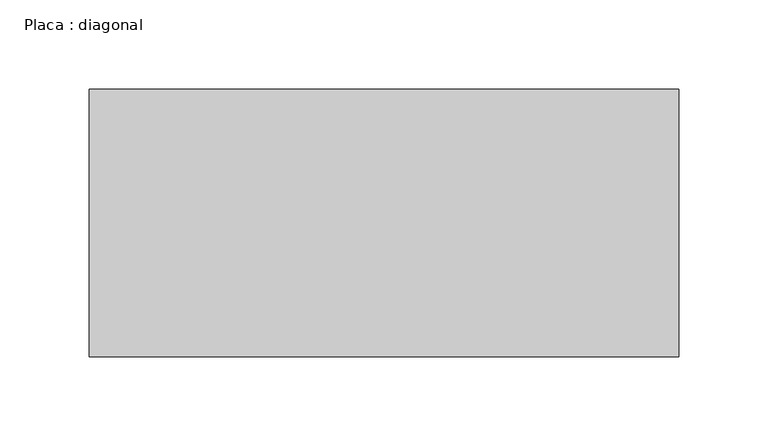
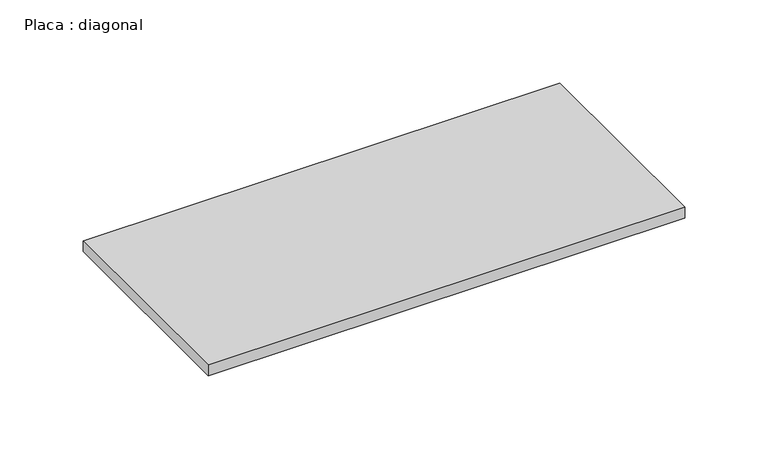
"""IFC4 building model written with IfcOpenShell, lengths in millimetres: beam geometry, Placa : diagonal."""

from ifc_helpers import new_model, si_unit, frame, origin, place, context, project, spatial, polyline, outline, extrude, source, transform, mapped, element, save


def placa_diagonal_d62ed6d6(model_context):
    return source(origin(), model_context, "Body", "SweptSolid", [
        extrude(outline(polyline([(165.4962734, 75.0), (165.4962734, -75.0), (-165.170522, -75.0), (-165.170522, 75.0), (165.4962734, 75.0)])), frame((0.0, 0.0, -4.0), z_axis=(0.0, 0.0, 1.0), x_axis=(1.0, 0.0, 0.0)), (0.0, 0.0, 1.0), 8.0),
    ])


if __name__ == "__main__":
    model = new_model("IFC4")
    model_context = context("Model", 3, world=origin())
    ifc_project = project(units=[si_unit("LENGTHUNIT", "METRE", prefix="MILLI")], contexts=[model_context])
    site = spatial("IfcSite", under=ifc_project)
    building = spatial("IfcBuilding", under=site)
    placement = place(None, origin())
    placa_diagonal_shape = placa_diagonal_d62ed6d6(model_context)
    element("IfcBeam", 1, ObjectType="Placa : diagonal", at=placement, inside=building, context=model_context, shape_type="MappedRepresentation", body=[
        mapped(placa_diagonal_shape, transform((0.0, 0.0, 0.0), x_axis=(1.0, 0.0, 0.0), y_axis=(0.0, 1.0, 0.0), z_axis=(0.0, 0.0, 1.0))),
    ])
    save(model, "model.ifc")

# Revit data of these elements
# Type "Placa : diagonal"
#   W = 0
#   Length [instance default] = 1.50 m
#   b = 0.15 m
#   d = 0.008 m
#   A = 0 m²
#   Structural Material [instance default] = Aço, 45-345
# Element 1 (IfcBeam, "Placa : diagonal")
#   Materials on its faces: "Aço, 45-345"
# Materials
#   "Aço, 45-345": class "Metal", colour RGB 247 247 247, transparency 0, Description = "Aço 345 MPa", Cost = 0
